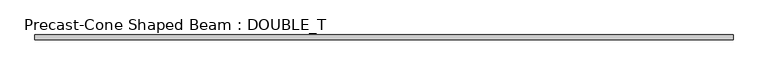
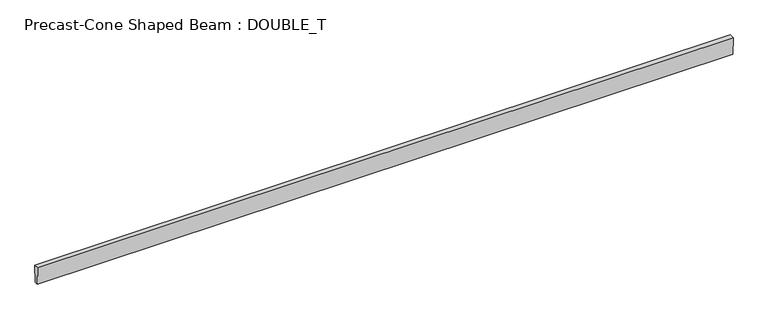
"""IFC4 building model written with IfcOpenShell, lengths in millimetres: beam geometry, Precast-Cone Shaped Beam : DOUBLE_T."""

from ifc_helpers import new_model, si_unit, frame, origin, place, context, project, spatial, polyline, outline, extrude, source, transform, mapped, element, save


def precast_cone_shaped_beam_double_t_5031dc9e(model_context):
    return source(origin(), model_context, "Body", "SweptSolid", [
        extrude(outline(polyline([(-50.8, -228.6), (-63.5, 228.6), (63.5, 228.6), (50.8, -228.6), (-50.8, -228.6)])), frame((-8915.4, 0.0, 0.0), z_axis=(1.0, 0.0, 0.0), x_axis=(0.0, 1.0, 0.0)), (0.0, 0.0, 1.0), 17983.2),
    ])


if __name__ == "__main__":
    model = new_model("IFC4")
    model_context = context("Model", 3, world=origin())
    ifc_project = project(units=[si_unit("LENGTHUNIT", "METRE", prefix="MILLI")], contexts=[model_context])
    site = spatial("IfcSite", under=ifc_project)
    building = spatial("IfcBuilding", under=site)
    placement = place(None, origin())
    precast_cone_shaped_beam_double_t_shape = precast_cone_shaped_beam_double_t_5031dc9e(model_context)
    element("IfcBeam", 1, ObjectType="Precast-Cone Shaped Beam : DOUBLE_T", at=placement, inside=building, context=model_context, shape_type="MappedRepresentation", body=[
        mapped(precast_cone_shaped_beam_double_t_shape, transform((0.0, 0.0, 0.0), x_axis=(1.0, 0.0, 0.0), y_axis=(0.0, 1.0, 0.0), z_axis=(0.0, 0.0, 1.0))),
    ])
    save(model, "model.ifc")

# Revit data of these elements
# Type "Precast-Cone Shaped Beam : DOUBLE_T"
#   Top Width = 0' - 5"
#   Tie Rod Weight [instance default] = 30
#   Tie Rod W [instance default] = 0.0660938 kip
#   Single Rebar Weight [instance default] = 50
#   Single Rebar W [instance default] = 0.110156 kip
#   Rebar Grids Weight [instance default] = 100
#   Rebar Grids W [instance default] = 0.220313 kip
#   Depth = 1' - 6"
#   Bottom Width = 0' - 4"
#   Length [instance default] = 5' - 0"
#   Structural Material [instance default] = Concrete, Precast
#   Assembly Code = ""
# Element 1 (IfcBeam, "Precast-Cone Shaped Beam : DOUBLE_T")
#   Length = 59' - 6"
#   Structural Material = Concrete - Precast Concrete - Normal Weight Concrete - 5 ksi
#   Materials on its faces: "Concrete - Precast Concrete - Normal Weight Concrete - 5 ksi"
# Materials
#   "Concrete, Precast": class "Concrete", colour RGB 198 187 187, transparency 0, Description = "Precast concrete", Cost = 0
#   "Concrete - Precast Concrete - Normal Weight Concrete - 5 ksi": class "Concrete", colour RGB 198 187 187, transparency 0, Cost = 0
